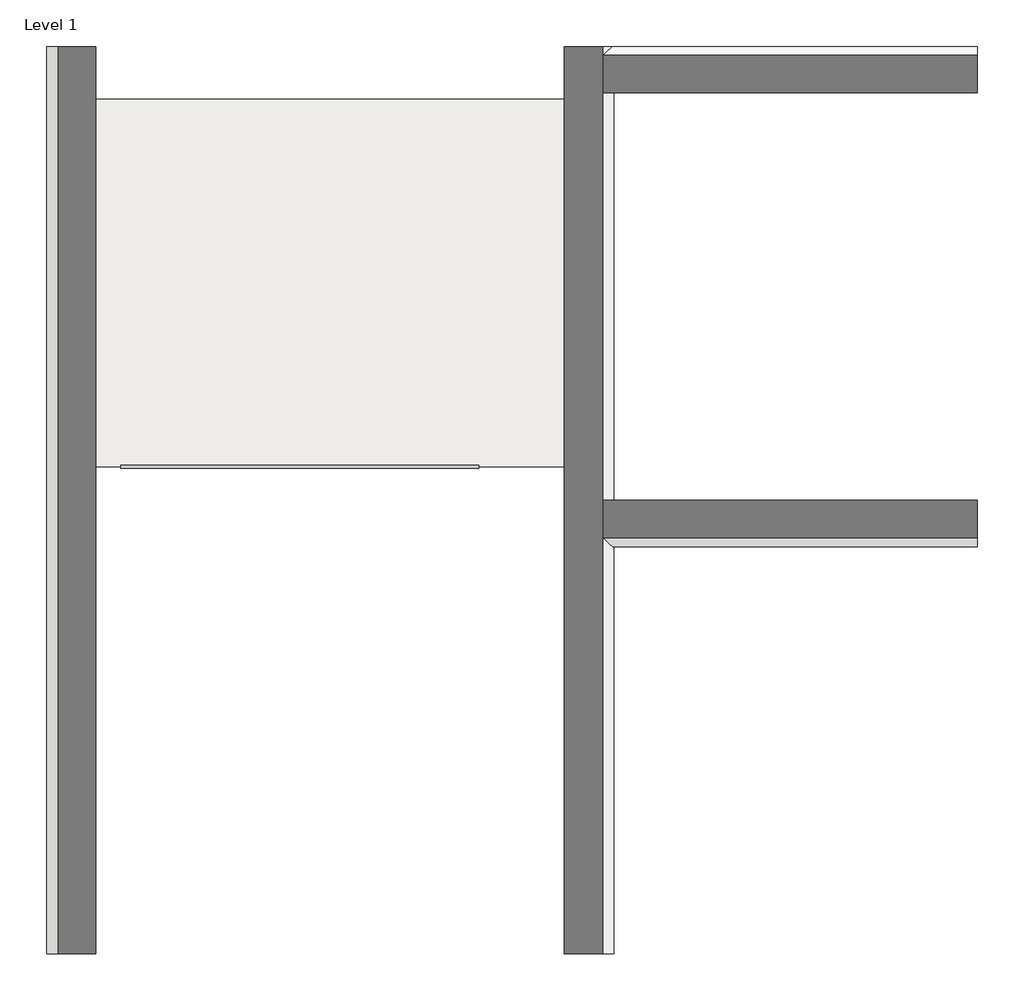
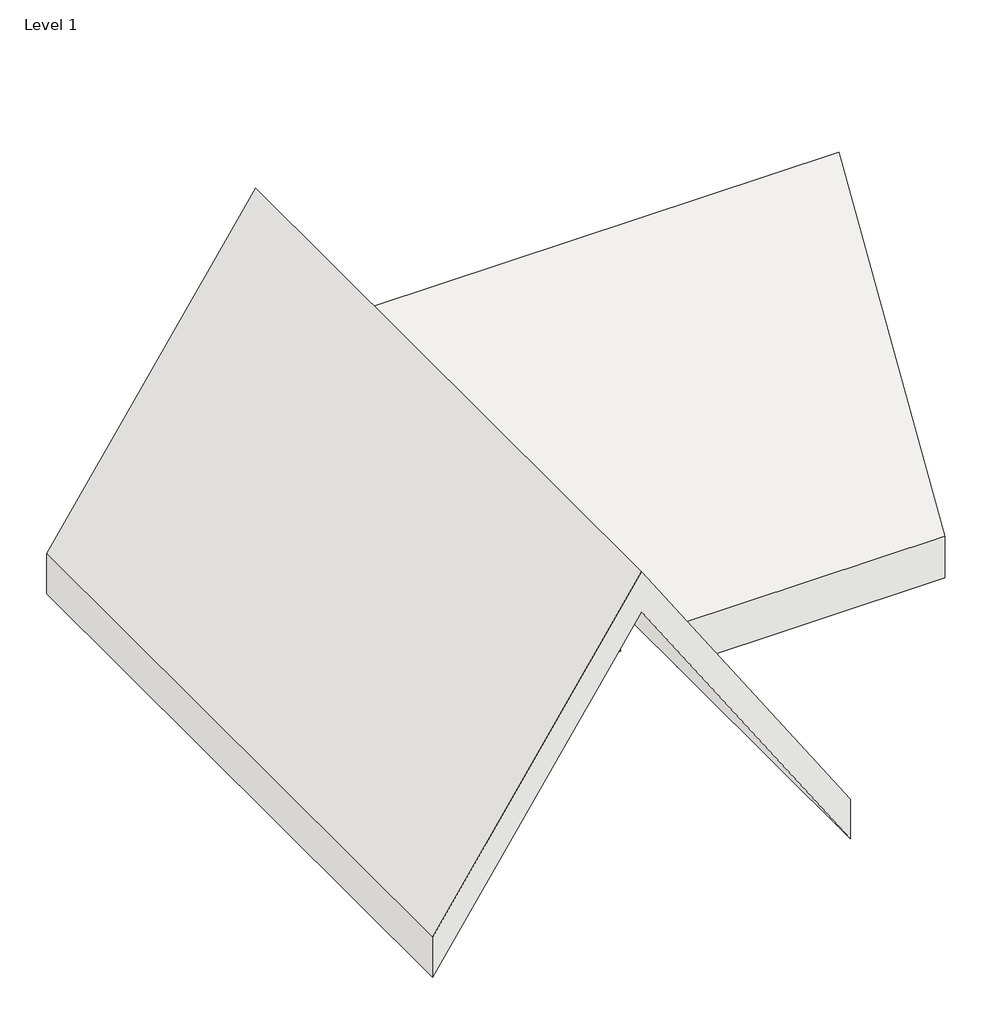
# One storey: 2 roofs, 1 railing, 1 slab.
"""IFC4 building model written with IfcOpenShell, lengths in millimetres."""

from ifc_helpers import new_model, si_unit, frame, origin, place, context, project, spatial, polyline, outline, extrude, faceted_brep, element, save

model = new_model("IFC4")

# Units and contexts
model_context = context("Model", 3, world=origin())
ifc_project = project(units=[si_unit("LENGTHUNIT", "METRE", prefix="MILLI")], contexts=[model_context])

# Site, building, storey
site = spatial("IfcSite", under=ifc_project)
building = spatial("IfcBuilding", under=site)
storey = spatial("IfcBuildingStorey", under=building, Name="Level 1", Elevation=3000.0)

# Railing
placement = place(None, origin())
element("IfcRailing", 1, ObjectType="1100mm", at=placement, inside=storey, context=model_context, shape_type="SweptSolid", body=[
    extrude(outline(polyline([(-3655.436416, -149.3443677), (-3655.436416, -99.3443677), (2144.563584, -99.3443677), (2144.563584, -149.3443677), (-3655.436416, -149.3443677)])), frame((0.0, 0.0, 4050.0), z_axis=(0.0, 0.0, 1.0), x_axis=(1.0, 0.0, 0.0)), (0.0, 0.0, 1.0), 50.0),
    extrude(outline(polyline([(2107.063584, -136.8443677), (2107.063584, -111.8443677), (2132.063584, -111.8443677), (2132.063584, -136.8443677), (2107.063584, -136.8443677)])), frame((0.0, 0.0, 3000.0), z_axis=(0.0, 0.0, 1.0), x_axis=(1.0, 0.0, 0.0)), (0.0, 0.0, 1.0), 1050.0),
    extrude(outline(polyline([(1832.063584, -136.8443677), (1832.063584, -111.8443677), (1857.063584, -111.8443677), (1857.063584, -136.8443677), (1832.063584, -136.8443677)])), frame((0.0, 0.0, 3000.0), z_axis=(0.0, 0.0, 1.0), x_axis=(1.0, 0.0, 0.0)), (0.0, 0.0, 1.0), 1050.0),
    extrude(outline(polyline([(1557.063584, -136.8443677), (1557.063584, -111.8443677), (1582.063584, -111.8443677), (1582.063584, -136.8443677), (1557.063584, -136.8443677)])), frame((0.0, 0.0, 3000.0), z_axis=(0.0, 0.0, 1.0), x_axis=(1.0, 0.0, 0.0)), (0.0, 0.0, 1.0), 1050.0),
    extrude(outline(polyline([(1282.063584, -136.8443677), (1282.063584, -111.8443677), (1307.063584, -111.8443677), (1307.063584, -136.8443677), (1282.063584, -136.8443677)])), frame((0.0, 0.0, 3000.0), z_axis=(0.0, 0.0, 1.0), x_axis=(1.0, 0.0, 0.0)), (0.0, 0.0, 1.0), 1050.0),
    extrude(outline(polyline([(1007.063584, -136.8443677), (1007.063584, -111.8443677), (1032.063584, -111.8443677), (1032.063584, -136.8443677), (1007.063584, -136.8443677)])), frame((0.0, 0.0, 3000.0), z_axis=(0.0, 0.0, 1.0), x_axis=(1.0, 0.0, 0.0)), (0.0, 0.0, 1.0), 1050.0),
    extrude(outline(polyline([(732.063584, -136.8443677), (732.063584, -111.8443677), (757.063584, -111.8443677), (757.063584, -136.8443677), (732.063584, -136.8443677)])), frame((0.0, 0.0, 3000.0), z_axis=(0.0, 0.0, 1.0), x_axis=(1.0, 0.0, 0.0)), (0.0, 0.0, 1.0), 1050.0),
    extrude(outline(polyline([(457.063584, -136.8443677), (457.063584, -111.8443677), (482.063584, -111.8443677), (482.063584, -136.8443677), (457.063584, -136.8443677)])), frame((0.0, 0.0, 3000.0), z_axis=(0.0, 0.0, 1.0), x_axis=(1.0, 0.0, 0.0)), (0.0, 0.0, 1.0), 1050.0),
    extrude(outline(polyline([(182.063584, -136.8443677), (182.063584, -111.8443677), (207.063584, -111.8443677), (207.063584, -136.8443677), (182.063584, -136.8443677)])), frame((0.0, 0.0, 3000.0), z_axis=(0.0, 0.0, 1.0), x_axis=(1.0, 0.0, 0.0)), (0.0, 0.0, 1.0), 1050.0),
    extrude(outline(polyline([(-92.936416, -136.8443677), (-92.936416, -111.8443677), (-67.936416, -111.8443677), (-67.936416, -136.8443677), (-92.936416, -136.8443677)])), frame((0.0, 0.0, 3000.0), z_axis=(0.0, 0.0, 1.0), x_axis=(1.0, 0.0, 0.0)), (0.0, 0.0, 1.0), 1050.0),
    extrude(outline(polyline([(-367.936416, -136.8443677), (-367.936416, -111.8443677), (-342.936416, -111.8443677), (-342.936416, -136.8443677), (-367.936416, -136.8443677)])), frame((0.0, 0.0, 3000.0), z_axis=(0.0, 0.0, 1.0), x_axis=(1.0, 0.0, 0.0)), (0.0, 0.0, 1.0), 1050.0),
    extrude(outline(polyline([(-642.936416, -136.8443677), (-642.936416, -111.8443677), (-617.936416, -111.8443677), (-617.936416, -136.8443677), (-642.936416, -136.8443677)])), frame((0.0, 0.0, 3000.0), z_axis=(0.0, 0.0, 1.0), x_axis=(1.0, 0.0, 0.0)), (0.0, 0.0, 1.0), 1050.0),
    extrude(outline(polyline([(-917.936416, -136.8443677), (-917.936416, -111.8443677), (-892.936416, -111.8443677), (-892.936416, -136.8443677), (-917.936416, -136.8443677)])), frame((0.0, 0.0, 3000.0), z_axis=(0.0, 0.0, 1.0), x_axis=(1.0, 0.0, 0.0)), (0.0, 0.0, 1.0), 1050.0),
    extrude(outline(polyline([(-1192.936416, -136.8443677), (-1192.936416, -111.8443677), (-1167.936416, -111.8443677), (-1167.936416, -136.8443677), (-1192.936416, -136.8443677)])), frame((0.0, 0.0, 3000.0), z_axis=(0.0, 0.0, 1.0), x_axis=(1.0, 0.0, 0.0)), (0.0, 0.0, 1.0), 1050.0),
    extrude(outline(polyline([(-1467.936416, -136.8443677), (-1467.936416, -111.8443677), (-1442.936416, -111.8443677), (-1442.936416, -136.8443677), (-1467.936416, -136.8443677)])), frame((0.0, 0.0, 3000.0), z_axis=(0.0, 0.0, 1.0), x_axis=(1.0, 0.0, 0.0)), (0.0, 0.0, 1.0), 1050.0),
    extrude(outline(polyline([(-1742.936416, -136.8443677), (-1742.936416, -111.8443677), (-1717.936416, -111.8443677), (-1717.936416, -136.8443677), (-1742.936416, -136.8443677)])), frame((0.0, 0.0, 3000.0), z_axis=(0.0, 0.0, 1.0), x_axis=(1.0, 0.0, 0.0)), (0.0, 0.0, 1.0), 1050.0),
    extrude(outline(polyline([(-2017.936416, -136.8443677), (-2017.936416, -111.8443677), (-1992.936416, -111.8443677), (-1992.936416, -136.8443677), (-2017.936416, -136.8443677)])), frame((0.0, 0.0, 3000.0), z_axis=(0.0, 0.0, 1.0), x_axis=(1.0, 0.0, 0.0)), (0.0, 0.0, 1.0), 1050.0),
    extrude(outline(polyline([(-2292.936416, -136.8443677), (-2292.936416, -111.8443677), (-2267.936416, -111.8443677), (-2267.936416, -136.8443677), (-2292.936416, -136.8443677)])), frame((0.0, 0.0, 3000.0), z_axis=(0.0, 0.0, 1.0), x_axis=(1.0, 0.0, 0.0)), (0.0, 0.0, 1.0), 1050.0),
    extrude(outline(polyline([(-2567.936416, -136.8443677), (-2567.936416, -111.8443677), (-2542.936416, -111.8443677), (-2542.936416, -136.8443677), (-2567.936416, -136.8443677)])), frame((0.0, 0.0, 3000.0), z_axis=(0.0, 0.0, 1.0), x_axis=(1.0, 0.0, 0.0)), (0.0, 0.0, 1.0), 1050.0),
    extrude(outline(polyline([(-2842.936416, -136.8443677), (-2842.936416, -111.8443677), (-2817.936416, -111.8443677), (-2817.936416, -136.8443677), (-2842.936416, -136.8443677)])), frame((0.0, 0.0, 3000.0), z_axis=(0.0, 0.0, 1.0), x_axis=(1.0, 0.0, 0.0)), (0.0, 0.0, 1.0), 1050.0),
    extrude(outline(polyline([(-3117.936416, -136.8443677), (-3117.936416, -111.8443677), (-3092.936416, -111.8443677), (-3092.936416, -136.8443677), (-3117.936416, -136.8443677)])), frame((0.0, 0.0, 3000.0), z_axis=(0.0, 0.0, 1.0), x_axis=(1.0, 0.0, 0.0)), (0.0, 0.0, 1.0), 1050.0),
    extrude(outline(polyline([(-3392.936416, -136.8443677), (-3392.936416, -111.8443677), (-3367.936416, -111.8443677), (-3367.936416, -136.8443677), (-3392.936416, -136.8443677)])), frame((0.0, 0.0, 3000.0), z_axis=(0.0, 0.0, 1.0), x_axis=(1.0, 0.0, 0.0)), (0.0, 0.0, 1.0), 1050.0),
    extrude(outline(polyline([(2119.563584, -136.8443677), (2119.563584, -111.8443677), (2144.563584, -111.8443677), (2144.563584, -136.8443677), (2119.563584, -136.8443677)])), frame((0.0, 0.0, 3000.0), z_axis=(0.0, 0.0, 1.0), x_axis=(1.0, 0.0, 0.0)), (0.0, 0.0, 1.0), 1050.0),
    extrude(outline(polyline([(-3655.436416, -136.8443677), (-3655.436416, -111.8443677), (-3630.436416, -111.8443677), (-3630.436416, -136.8443677), (-3655.436416, -136.8443677)])), frame((0.0, 0.0, 3000.0), z_axis=(0.0, 0.0, 1.0), x_axis=(1.0, 0.0, 0.0)), (0.0, 0.0, 1.0), 1050.0),
])

# Roofs
element("IfcRoof", 2, ObjectType="Roof_Pitched-50SS-220Ins-20MPan-225Purl", at=placement, inside=storey, context=model_context, shape_type="SweptSolid", body=[
    extrude(outline(polyline([(3928.3411011, 4334.563584), (10819.8936519, -260.436416), (3928.3411011, -4855.436416), (3000.0, -4855.436416), (9891.5525508, -260.436416), (3000.0, 4334.563584), (3928.3411011, 4334.563584)])), frame((0.0, -8014.3443677, 0.0), z_axis=(0.0, 1.0, 0.0), x_axis=(0.0, 0.0, 1.0)), (0.0, 0.0, 1.0), 14700.0),
])
element("IfcRoof", 3, ObjectType="Roof_Pitched-50SS-220Ins-20MPan-225Purl", at=placement, inside=storey, context=model_context, shape_type="Brep", body=[
    faceted_brep([(642.4602323, 2635.6556323, 9465.7348488), (4334.563584, 6104.1623377, 3928.3411011), (4334.563584, 6685.6556323, 3000.0), (10224.563584, 6685.6556323, 3000.0), (10224.563584, 2635.6556323, 9465.7348488), (10224.563584, -1414.3443677, 3000.0), (4334.563584, -1414.3443677, 3000.0), (4334.563584, -832.851073, 3928.3411011), (4306.6789551, 6685.6556323, 3970.1622948), (-4.4035494, 2635.6556323, 10435.8971437), (10224.563584, 2635.6556323, 10435.8971437), (10224.563584, 6685.6556323, 3970.1622948), (4306.6789551, -1414.3443677, 3970.1622948), (10224.563584, -1414.3443677, 3970.1622948), (4334.563584, -1414.3443677, 3928.3411011), (4334.563584, 6685.6556323, 3928.3411011)], [[[0, 1, 2, 3, 4]], [[5, 6, 7, 0, 4]], [[8, 9, 10, 11]], [[12, 13, 10, 9]], [[5, 13, 12, 14, 6]], [[2, 15, 8, 11, 3]], [[11, 10, 13, 5, 4, 3]], [[12, 9, 8, 15, 1, 0, 7, 14]], [[7, 6, 14]], [[15, 2, 1]]]),
])

# Slab
element("IfcSlab", 4, ObjectType="Floor_Timber_22Cbd-225Joist", at=placement, inside=storey, context=model_context, shape_type="SweptSolid", body=[
    extrude(outline(polyline([(3834.563584, 5830.6556323), (3834.563584, -124.3443677), (-4500.436416, -124.3443677), (-4500.436416, 5830.6556323), (3834.563584, 5830.6556323)])), frame((0.0, 0.0, 2753.0), z_axis=(0.0, 0.0, 1.0), x_axis=(1.0, 0.0, 0.0)), (0.0, 0.0, 1.0), 247.0),
])

save(model, "model.ifc")

# Revit data of these elements
# Project information
#   Project Issue Date = "Issue Date"
#   Project Status = "Project Status"
#   Client Name = "Owner"
#   Project Address = "Enter address here"
#   Project Name = "Project Name"
#   Project Number = "Project Number"
# Type "1100mm"
#   built-in parameter 1008612 = 0.019685 (stored number, unit not read)
#   built-in parameter 1008611 = 0.019685 (stored number, unit not read)
#   built-in parameter 1008609 = 0.902231 (stored number, unit not read)
#   built-in parameter 1008604 = 0.19685 (stored number, unit not read)
#   built-in parameter 1008603 = 0.164042 (stored number, unit not read)
#   Railing Height = 1100 mm
#   built-in parameter 1008630 = 2
#   built-in parameter 1008610 = 2
#   built-in parameter 1008608 = 1
#   built-in parameter 1008618 = Baluster_Square : 25mm
# Type "Roof_Pitched-50SS-220Ins-20MPan-225Purl"
#   Layers, outside or top first: 50 mm "Roofing, Standing Seam" (function 5); 220 mm "Rigid insulation" (function 3); 20 mm "Metal Panel" (function 4); 225 mm "Steel Purlins" (function 1)
# Type "Floor_Timber_22Cbd-225Joist"
#   Function = 0
#   Layers, outside or top first: 22 mm "Wood Sheathing, Chipboard" (function 5); 225 mm "Structure, Timber Joist/Rafter Layer" (function 1)
# Element 1 (IfcRailing, "1100mm")
#   Phase Created = New Construction
# Element 2 (IfcRoof, "Roof_Pitched-50SS-220Ins-20MPan-225Purl")
#   built-in parameter 1001705 = 35.4983 (stored number, unit not read)
#   built-in parameter 1001710 = 33615
#   Phase Created = New Construction
#   Materials on its faces: "Steel Purlins", "Roofing, Standing Seam"
# Element 3 (IfcRoof, "Roof_Pitched-50SS-220Ins-20MPan-225Purl")
#   built-in parameter 1001705 = 34.2385 (stored number, unit not read)
#   built-in parameter 1001710 = 33615
#   Phase Created = New Construction
#   Materials on its faces: "Steel Purlins", "Roofing, Standing Seam"
# Element 4 (IfcSlab, "Floor_Timber_22Cbd-225Joist")
#   Height Offset From Level = 0 mm
#   Phase Created = New Construction
#   Materials on its faces: "Structure, Timber Joist/Rafter Layer", "Wood Sheathing, Chipboard"
# Materials
#   "Roofing, Standing Seam": class "Metal", colour RGB 247 247 247, transparency 0, Description = "Aluminum standing seam roofing", Cost = 0
#   "Rigid insulation": class "Generic", colour RGB 127 127 127, transparency 0, Description = "Rigid foam insulation board", Cost = 0
#   "Metal Panel": class "Metal", colour RGB 247 247 247, transparency 0, Description = "Stainless steel panels", Cost = 0
#   "Steel Purlins": class "Metal", colour RGB 247 247 247, transparency 0, Description = "Light gauge steel purlins", Cost = 0
#   "Wood Sheathing, Chipboard": class "Wood", colour RGB 127 127 127, transparency 0, Description = "Particleboard sheathing", Cost = 0
#   "Structure, Timber Joist/Rafter Layer": class "Wood", colour RGB 127 127 127, transparency 0, Description = "Timber framing, thermal airspace", Cost = 0
